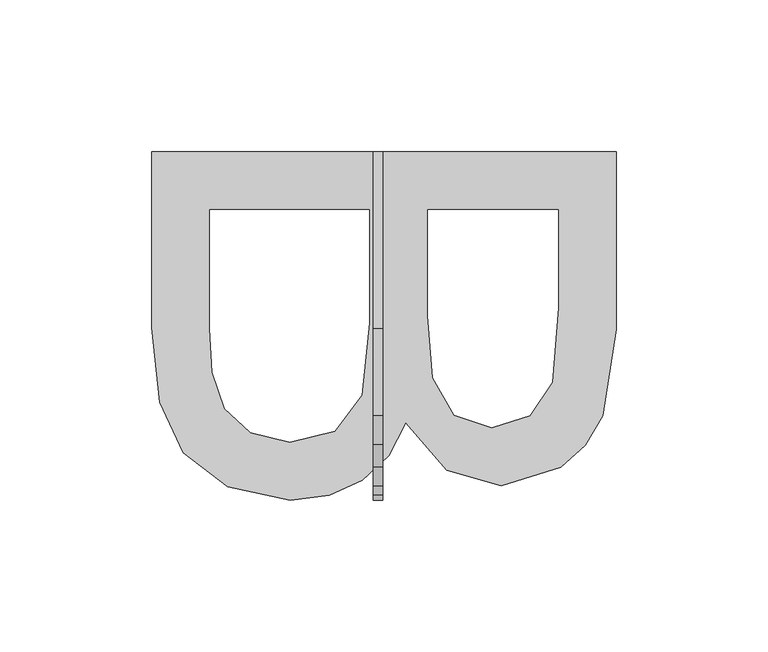
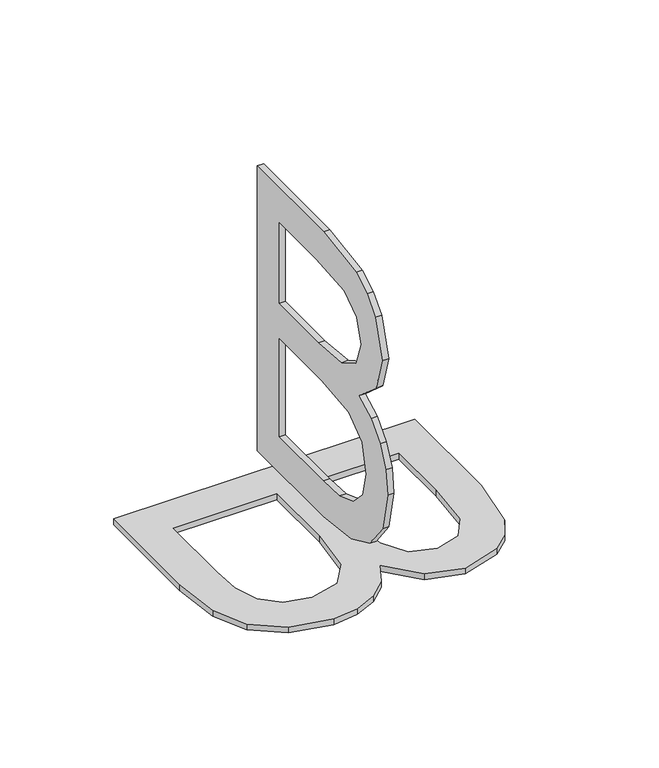
"""IFC4 building model written with IfcOpenShell, lengths in millimetres: proxy geometry, Grid Number2_FedEx : Grid Number2_FedEx."""

from ifc_helpers import new_model, si_unit, frame, origin, origin_with_axes, place, context, project, spatial, polyline, outline, extrude, source, transform, mapped, element, save


def entourage_76d14982(model_context):
    return source(origin(), model_context, "Body", "SweptSolid", [
        extrude(outline(polyline([(-184.2739267, 276.3432839), (-31.1785101, 276.3432839), (-31.1785101, 217.9233288), (-35.6824158, 189.3113802), (-41.3963957, 179.6961957), (-49.5305241, 172.4170618), (-69.1159729, 166.3059532), (-87.0007769, 171.4452647), (-100.5498707, 186.9753295), (-106.2124576, 176.1313823), (-114.8278124, 168.1187285), (-125.825939, 163.1709732), (-138.6368409, 161.5217214), (-159.2127752, 166.0256271), (-173.864485, 177.1826051), (-181.6388616, 193.8339743), (-184.2739267, 218.3718505), (-184.2739267, 276.3432839)]), holes=[polyline([(-93.3735231, 257.2063569), (-93.3735231, 222.2590388), (-91.7289434, 201.8513002), (-84.6460378, 189.5730179), (-72.1808714, 185.4428803), (-59.6970166, 189.2926918), (-52.3150965, 200.318851), (-50.3154372, 224.9127924), (-50.3154372, 257.2063569), (-93.3735231, 257.2063569)]), polyline([(-165.1369997, 257.2063569), (-165.1369997, 217.9607056), (-164.3894634, 203.7575175), (-160.221949, 191.7408729), (-151.7187246, 183.7796122), (-138.8237249, 180.6586485), (-123.9477543, 184.321576), (-115.0707617, 196.1887134), (-112.5104502, 219.8295462), (-112.5104502, 257.2063569), (-165.1369997, 257.2063569)])]), origin_with_axes(), (0.0, 0.0, 1.0), 3.175),
        extrude(outline(polyline([(276.3432839, 14.2382753), (218.3718505, 14.2382753), (193.8339743, 16.8733405), (177.1826051, 24.6477171), (166.0256271, 39.2994269), (161.5217214, 59.8753612), (163.1709732, 72.6862631), (168.1187285, 83.6843896), (176.1313823, 92.2997445), (186.9753295, 97.9623313), (171.4452647, 111.5114252), (166.3059532, 129.3962291), (172.4170618, 148.9816779), (179.6961957, 157.1158063), (189.3113802, 162.8297863), (217.9233288, 167.333692), (276.3432839, 167.333692), (276.3432839, 14.2382753)]), holes=[polyline([(257.2063569, 33.3752024), (257.2063569, 86.0017519), (219.8295462, 86.0017519), (196.1887134, 83.4414403), (184.321576, 74.5644478), (180.6586485, 59.6884771), (183.7796122, 46.7934774), (191.7408729, 38.290253), (203.7575175, 34.1227386), (217.9607056, 33.3752024), (257.2063569, 33.3752024)]), polyline([(257.2063569, 105.138679), (257.2063569, 148.1967649), (224.9127924, 148.1967649), (200.318851, 146.1971055), (189.2926918, 138.8151854), (185.4428803, 126.3313306), (189.5730179, 113.8661643), (201.8513002, 106.7832586), (222.2590388, 105.138679), (257.2063569, 105.138679)])]), frame((-111.2489267, 0.0, 0.0), z_axis=(1.0, 0.0, 0.0), x_axis=(0.0, 1.0, 0.0)), (0.0, 0.0, 1.0), 3.175),
    ])


if __name__ == "__main__":
    model = new_model("IFC4")
    model_context = context("Model", 3, world=origin())
    ifc_project = project(units=[si_unit("LENGTHUNIT", "METRE", prefix="MILLI")], contexts=[model_context])
    site = spatial("IfcSite", under=ifc_project)
    building = spatial("IfcBuilding", under=site)
    placement = place(None, origin())
    entourage_shape = entourage_76d14982(model_context)
    element("IfcBuildingElementProxy", 1, Name="Grid Number2_FedEx : Grid Number2_FedEx", ObjectType="Grid Number2_FedEx : Grid Number2_FedEx", at=placement, inside=building, context=model_context, shape_type="MappedRepresentation", body=[
        mapped(entourage_shape, transform((0.0, 0.0, 0.0), x_axis=(1.0, 0.0, 0.0), y_axis=(0.0, 1.0, 0.0), z_axis=(0.0, 0.0, 1.0))),
    ])
    save(model, "model.ifc")

# Revit data of these elements
# Type "Grid Number2_FedEx : Grid Number2_FedEx"
#   Grid [instance default] = "S"
#   Label Width [instance default] = 1' - 0"
#   Half Box Width2 [instance default] = 0' - 6.13846"
#   Half Box Width [instance default] = 0' - 6"
#   Robust [instance default] = yes
#   Height = 0
#   Assembly Code = ""
# Element 1 (IfcBuildingElementProxy, "Grid Number2_FedEx : Grid Number2_FedEx")
#   Grid = "B"
#   Robust = no
#   Materials on its faces: "Letter"
# Materials
#   "Letter": class "Unassigned", colour RGB 178 187 30, transparency 0, Comments = "Rendering appearance not upgraded "
